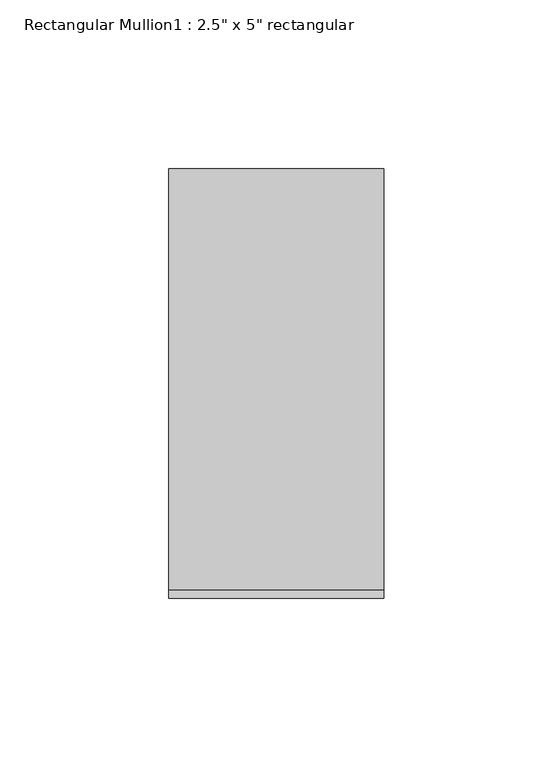
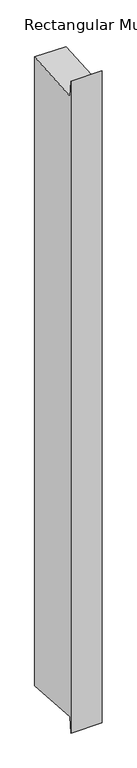
"""IFC4 building model written with IfcOpenShell, lengths in millimetres: member geometry."""

import ifcopenshell
import ifcopenshell.guid

model = None  # the IFC model being written
_history = None  # IfcOwnerHistory: only IFC2X3 demands one
_inside = {}  # id of a spatial element -> (the spatial element, [elements in it])
_under = {}  # id of a project, library or spatial element -> (it, [spatial elements below it])
_declared = {}  # id of a project -> (the project, [libraries it declares])
_typed = {}  # id of a type object -> (the type object, [elements of that type])
_made_of = {}  # id of a material, layer set ... -> (it, [elements and type objects made of it])


def new_model(schema):
    """Start an empty IFC model of exactly this schema.

    Asked for "IFC4X3", IfcOpenShell would pick the latest addendum, in which some entities
    have other attributes; the version numbers below select the first issue.
    IFC2X3 requires an IfcOwnerHistory on every rooted entity: one is made here for all.
    """
    global model, _history
    if schema == "IFC4X3":
        model = ifcopenshell.file(schema_version=(4, 3, 0, 0))
    else:
        model = ifcopenshell.file(schema=schema)
    _inside.clear()
    _under.clear()
    _declared.clear()
    _typed.clear()
    _made_of.clear()
    _history = None
    if model.schema == "IFC2X3":
        org = make("IfcOrganization", Name="unknown")
        user = make(
            "IfcPersonAndOrganization",
            ThePerson=make("IfcPerson", FamilyName="unknown"),
            TheOrganization=org,
        )
        app = make(
            "IfcApplication",
            ApplicationDeveloper=org,
            Version="unknown",
            ApplicationFullName="unknown",
            ApplicationIdentifier="unknown",
        )
        _history = make(
            "IfcOwnerHistory",
            OwningUser=user,
            OwningApplication=app,
            ChangeAction="ADDED",
            CreationDate=0,
        )
    return model


def make(cls, **values):
    """One entity of the class cls with the attributes given. An attribute that is None is left unset."""
    return model.create_entity(
        cls, **{name: value for name, value in values.items() if value is not None}
    )


def rooted(cls, **values):
    """An entity with a GlobalId (a new one), such as an element, a storey or a relation."""
    return make(cls, GlobalId=ifcopenshell.guid.new(), OwnerHistory=_history, **values)


def si_unit(unit_type, name, prefix=None):
    """IfcSIUnit, for example si_unit("LENGTHUNIT", "METRE", prefix="MILLI")."""
    return make("IfcSIUnit", UnitType=unit_type, Prefix=prefix, Name=name)


def assignment(units):
    """IfcUnitAssignment: the units of a project."""
    return None if units is None else make("IfcUnitAssignment", Units=units)


def point(xyz):
    """IfcCartesianPoint."""
    return None if xyz is None else make("IfcCartesianPoint", Coordinates=xyz)


def direction(xyz):
    """IfcDirection."""
    return None if xyz is None else make("IfcDirection", DirectionRatios=xyz)


def frame(location, z_axis=None, x_axis=None):
    """IfcAxis2Placement3D, a coordinate frame: its origin and axes. An axis left out is left unset."""
    return make(
        "IfcAxis2Placement3D",
        Location=point(location),
        Axis=direction(z_axis),
        RefDirection=direction(x_axis),
    )


def origin():
    """The frame at (0, 0, 0) with its axes left unset."""
    return frame((0.0, 0.0, 0.0))


def place(relative_to, where):
    """IfcLocalPlacement: puts the frame where relative to a parent placement (None: the world)."""
    return make(
        "IfcLocalPlacement", PlacementRelTo=relative_to, RelativePlacement=where
    )


def context(
    kind, dimensions, precision=None, world=None, true_north=None, identifier=None
):
    """IfcGeometricRepresentationContext, for example the 3D "Model" context."""
    return make(
        "IfcGeometricRepresentationContext",
        ContextIdentifier=identifier,
        ContextType=kind,
        CoordinateSpaceDimension=dimensions,
        Precision=precision,
        WorldCoordinateSystem=world,
        TrueNorth=true_north,
    )


def project(units=None, contexts=None):
    """IfcProject with its units and contexts."""
    return rooted(
        "IfcProject",
        Name="project",
        RepresentationContexts=contexts,
        UnitsInContext=assignment(units),
    )


def spatial(cls, under=None, at=None, **own):
    """A site, building, storey or space (cls), placed at a placement, below another one or the project."""
    s = rooted(cls, ObjectPlacement=at, **own)
    if under is not None:
        _under.setdefault(under.id(), (under, []))[1].append(s)
    return s


def polyline(points):
    """IfcPolyline through the points."""
    return make("IfcPolyline", Points=[point(p) for p in points])


def outline(outer, holes=None, kind="AREA"):
    """IfcArbitraryClosedProfileDef: a profile drawn as a closed curve; with holes, ...WithVoids."""
    if holes is None:
        return make("IfcArbitraryClosedProfileDef", ProfileType=kind, OuterCurve=outer)
    return make(
        "IfcArbitraryProfileDefWithVoids",
        ProfileType=kind,
        OuterCurve=outer,
        InnerCurves=holes,
    )


def extrude(swept, where, along, depth):
    """IfcExtrudedAreaSolid: the profile swept, set in the frame where, extruded along a direction by depth."""
    return make(
        "IfcExtrudedAreaSolid",
        SweptArea=swept,
        Position=where,
        ExtrudedDirection=direction(along),
        Depth=depth,
    )


def shape(context_of_items, identifier, shape_type, items):
    """IfcShapeRepresentation: the items that make up one representation, for example the "Body"."""
    return make(
        "IfcShapeRepresentation",
        ContextOfItems=context_of_items,
        RepresentationIdentifier=identifier,
        RepresentationType=shape_type,
        Items=items,
    )


def source(mapping_origin, context_of_items, identifier, shape_type, items):
    """IfcRepresentationMap: a shape defined once, which mapped items show again and again."""
    return make(
        "IfcRepresentationMap",
        MappingOrigin=mapping_origin,
        MappedRepresentation=shape(context_of_items, identifier, shape_type, items),
    )


def transform(
    local_origin,
    x_axis=None,
    y_axis=None,
    z_axis=None,
    scale=None,
    scale2=None,
    scale3=None,
    uniform=True,
):
    """IfcCartesianTransformationOperator3D, or its non-uniform kind. x_axis, y_axis, z_axis: its Axis1, 2, 3."""
    if uniform:
        return make(
            "IfcCartesianTransformationOperator3D",
            Axis1=direction(x_axis),
            Axis2=direction(y_axis),
            LocalOrigin=point(local_origin),
            Scale=scale,
            Axis3=direction(z_axis),
        )
    return make(
        "IfcCartesianTransformationOperator3DnonUniform",
        Axis1=direction(x_axis),
        Axis2=direction(y_axis),
        LocalOrigin=point(local_origin),
        Scale=scale,
        Axis3=direction(z_axis),
        Scale2=scale2,
        Scale3=scale3,
    )


def mapped(mapping_source, mapping_target):
    """IfcMappedItem: shows the shape of a source again, moved by a transform."""
    return make(
        "IfcMappedItem", MappingSource=mapping_source, MappingTarget=mapping_target
    )


def made_of(thing, what):
    """Note that an element or type object is made of a material, layer set ...; save() writes the relation."""
    if what is not None:
        _made_of.setdefault(what.id(), (what, []))[1].append(thing)
    return thing


def element(
    cls,
    number,
    at=None,
    inside=None,
    cuts=None,
    type_object=None,
    material=None,
    context=None,
    identifier="Body",
    shape_type=None,
    held_by="IfcProductDefinitionShape",
    body=None,
    shapes=None,
    **own,
):
    """One element of the class cls, such as IfcWall. Its Tag is "e" and its number.

    at: its placement. inside: the storey or other place that contains it. cuts: it is an
    opening in that element (IfcRelVoidsElement). A single representation is given by context,
    identifier, shape_type and body (its items); several are given by shapes. held_by: the class
    of the entity that holds the representations. save() writes the other relations.
    """
    e = rooted(cls, Tag="e%d" % number, ObjectPlacement=at, **own)
    if body is not None:
        shapes = [shape(context, identifier, shape_type, body)]
    if shapes is not None:
        e.Representation = make(held_by, Representations=shapes)
    if inside is not None:
        _inside.setdefault(inside.id(), (inside, []))[1].append(e)
    if cuts is not None:
        rooted(
            "IfcRelVoidsElement", RelatingBuildingElement=cuts, RelatedOpeningElement=e
        )
    if type_object is not None:
        _typed.setdefault(type_object.id(), (type_object, []))[1].append(e)
    return made_of(e, material)


def aggregate(whole, parts):
    """IfcRelAggregates: a whole, such as a stair, and the parts it consists of."""
    return rooted("IfcRelAggregates", RelatingObject=whole, RelatedObjects=parts)


def save(model, path):
    """Write the relations noted so far, then the file.

    IfcRelAggregates (storeys below a building ...), IfcRelContainedInSpatialStructure (elements
    in a storey), IfcRelDefinesByType, IfcRelAssociatesMaterial and IfcRelDeclares: one each for
    every whole, place, type object, material and project.
    """
    for whole, parts in _under.values():
        aggregate(whole, parts)
    for where, things in _inside.values():
        rooted(
            "IfcRelContainedInSpatialStructure",
            RelatedElements=things,
            RelatingStructure=where,
        )
    for kind, things in _typed.values():
        rooted("IfcRelDefinesByType", RelatedObjects=things, RelatingType=kind)
    for what, things in _made_of.values():
        rooted("IfcRelAssociatesMaterial", RelatedObjects=things, RelatingMaterial=what)
    for by, libraries in _declared.values():
        rooted("IfcRelDeclares", RelatingContext=by, RelatedDefinitions=libraries)
    model.write(path)


def member_233ab79f(model_context):
    return source(origin(), model_context, "Body", "SweptSolid", [
        extrude(outline(polyline([(-63.5, 29.4471051), (-61.0333155, -4.5163328), (63.5, 4.5282284), (63.5, -1343.9489353), (-61.0333155, -1334.904374), (-63.5, -1368.8678119), (-63.5, 29.4471051)])), frame((-63.5, 0.0, 0.0), z_axis=(1.0, 0.0, 0.0), x_axis=(0.0, 1.0, 0.0)), (0.0, 0.0, 1.0), 63.5),
    ])


if __name__ == "__main__":
    model = new_model("IFC4")
    model_context = context("Model", 3, world=origin())
    ifc_project = project(units=[si_unit("LENGTHUNIT", "METRE", prefix="MILLI")], contexts=[model_context])
    site = spatial("IfcSite", under=ifc_project)
    building = spatial("IfcBuilding", under=site)
    placement = place(None, origin())
    member_shape = member_233ab79f(model_context)
    element("IfcMember", 1, ObjectType="Rectangular Mullion1 : 2.5\" x 5\" rectangular", at=placement, inside=building, context=model_context, shape_type="MappedRepresentation", body=[
        mapped(member_shape, transform((0.0, 0.0, 0.0), x_axis=(1.0, 0.0, 0.0), y_axis=(0.0, 1.0, 0.0), z_axis=(0.0, 0.0, 1.0))),
    ])
    save(model, "model.ifc")

# Revit data of these elements
# Type "Rectangular Mullion1 : 2.5\" x 5\" rectangular"
#   built-in parameter 1007304 = 0.416667 (stored number, unit not read)
#   built-in parameter 1007301 = 0.104167 (stored number, unit not read)
#   built-in parameter 1007300 = 0.104167 (stored number, unit not read)
# Element 1 (IfcMember, "Rectangular Mullion1 : 2.5\" x 5\" rectangular")
#   Materials on its faces: "support-frame"
# Materials
#   "support-frame": class "Unassigned", colour RGB 233 233 233, transparency 0, Cost = 0
